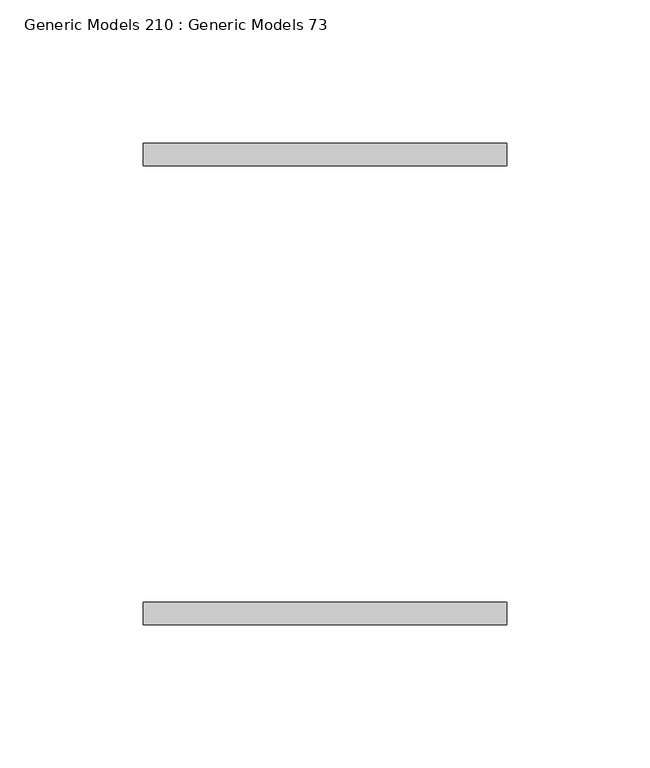
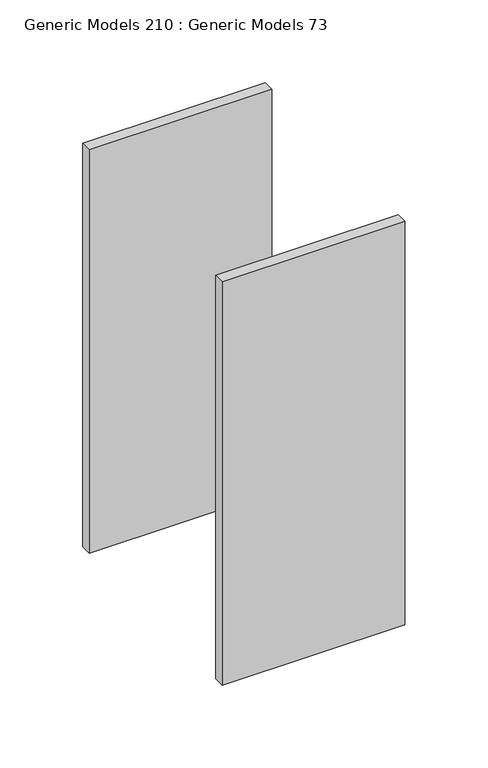
"""IFC4 building model written with IfcOpenShell, lengths in millimetres: proxy geometry, Generic Models 210 : Generic Models 73."""

from ifc_helpers import new_model, si_unit, frame, origin, place, context, project, spatial, polyline, outline, extrude, source, transform, mapped, element, save


def generic_models_210_generic_models_73_11dfd497(model_context):
    return source(origin(), model_context, "Body", "SweptSolid", [
        extrude(outline(polyline([(32053.2090778, 36491.5582942), (32053.2090778, 36483.6207942), (31926.2090778, 36483.6207942), (31926.2090778, 36491.5582942), (32053.2090778, 36491.5582942)])), frame((0.0, 0.0, 269146.3375), z_axis=(0.0, 0.0, 1.0), x_axis=(1.0, 0.0, 0.0)), (0.0, 0.0, 1.0), 296.8625),
        extrude(outline(polyline([(32053.2090778, 36331.2207942), (32053.2090778, 36323.2832942), (31926.2090778, 36323.2832942), (31926.2090778, 36331.2207942), (32053.2090778, 36331.2207942)])), frame((0.0, 0.0, 269146.3375), z_axis=(0.0, 0.0, 1.0), x_axis=(1.0, 0.0, 0.0)), (0.0, 0.0, 1.0), 296.8625),
    ])


if __name__ == "__main__":
    model = new_model("IFC4")
    model_context = context("Model", 3, world=origin())
    ifc_project = project(units=[si_unit("LENGTHUNIT", "METRE", prefix="MILLI")], contexts=[model_context])
    site = spatial("IfcSite", under=ifc_project)
    building = spatial("IfcBuilding", under=site)
    placement = place(None, origin())
    generic_models_210_generic_models_73_shape = generic_models_210_generic_models_73_11dfd497(model_context)
    element("IfcBuildingElementProxy", 1, Name="Generic Models 210 : Generic Models 73", ObjectType="Generic Models 210 : Generic Models 73", at=placement, inside=building, context=model_context, shape_type="MappedRepresentation", body=[
        mapped(generic_models_210_generic_models_73_shape, transform((0.0, 0.0, 0.0), x_axis=(1.0, 0.0, 0.0), y_axis=(0.0, 1.0, 0.0), z_axis=(0.0, 0.0, 1.0))),
    ])
    save(model, "model.ifc")

# Revit data of these elements
# Element 1 (IfcBuildingElementProxy, "Generic Models 210 : Generic Models 73")
#   Materials on its faces: "5/16 THICK GALV. SADDLE"
# Materials
#   "5/16 THICK GALV. SADDLE": class "Metal", colour RGB 199 199 199, transparency 0, Description = "Carbon steel", Cost = 0
